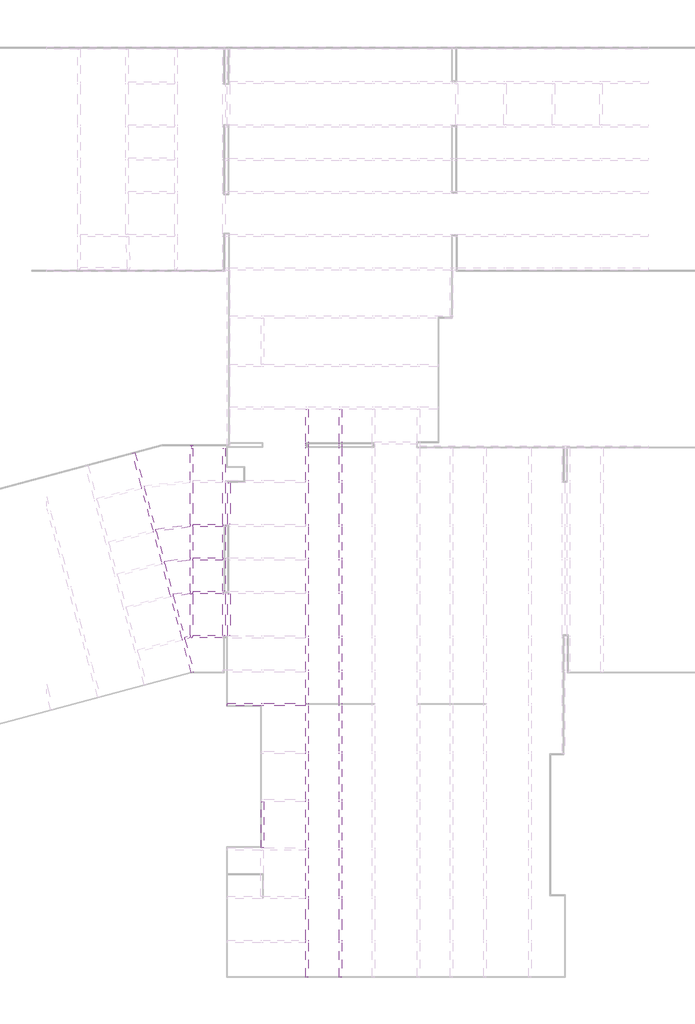
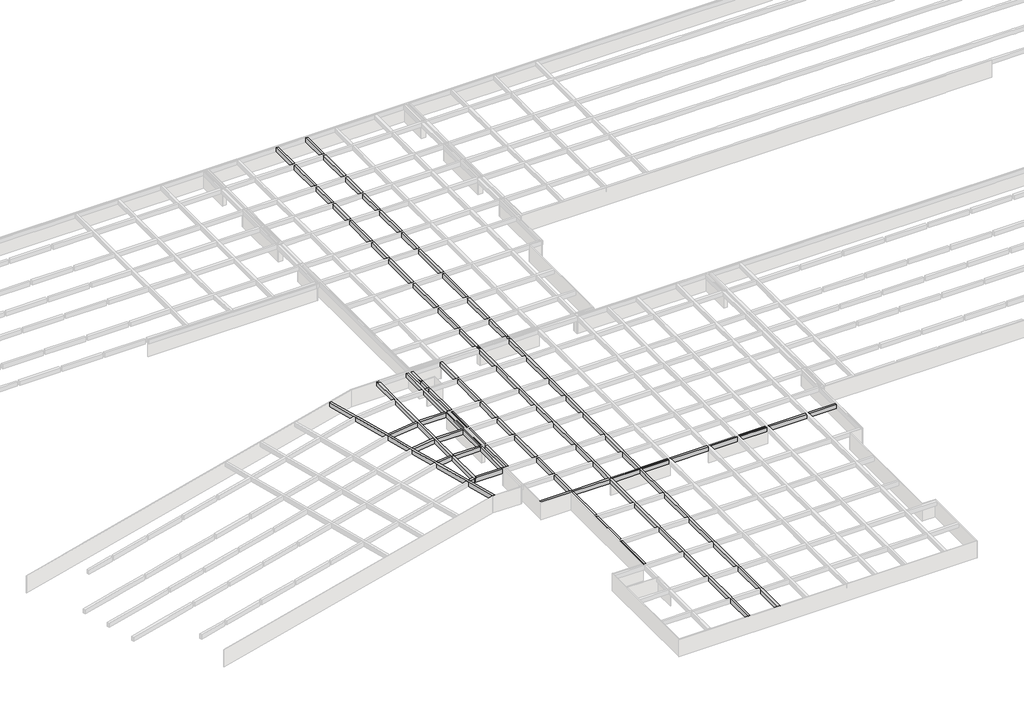
# One storey, part 7 of 14: 19 beams.
"""IFC4 building model written with IfcOpenShell, lengths in millimetres."""

import ifcopenshell
import ifcopenshell.guid

model = None  # the IFC model being written
_history = None  # IfcOwnerHistory: only IFC2X3 demands one
_inside = {}  # id of a spatial element -> (the spatial element, [elements in it])
_under = {}  # id of a project, library or spatial element -> (it, [spatial elements below it])
_declared = {}  # id of a project -> (the project, [libraries it declares])
_typed = {}  # id of a type object -> (the type object, [elements of that type])
_made_of = {}  # id of a material, layer set ... -> (it, [elements and type objects made of it])


def new_model(schema):
    """Start an empty IFC model of exactly this schema.

    Asked for "IFC4X3", IfcOpenShell would pick the latest addendum, in which some entities
    have other attributes; the version numbers below select the first issue.
    IFC2X3 requires an IfcOwnerHistory on every rooted entity: one is made here for all.
    """
    global model, _history
    if schema == "IFC4X3":
        model = ifcopenshell.file(schema_version=(4, 3, 0, 0))
    else:
        model = ifcopenshell.file(schema=schema)
    _inside.clear()
    _under.clear()
    _declared.clear()
    _typed.clear()
    _made_of.clear()
    _history = None
    if model.schema == "IFC2X3":
        org = make("IfcOrganization", Name="unknown")
        user = make(
            "IfcPersonAndOrganization",
            ThePerson=make("IfcPerson", FamilyName="unknown"),
            TheOrganization=org,
        )
        app = make(
            "IfcApplication",
            ApplicationDeveloper=org,
            Version="unknown",
            ApplicationFullName="unknown",
            ApplicationIdentifier="unknown",
        )
        _history = make(
            "IfcOwnerHistory",
            OwningUser=user,
            OwningApplication=app,
            ChangeAction="ADDED",
            CreationDate=0,
        )
    return model


def make(cls, **values):
    """One entity of the class cls with the attributes given. An attribute that is None is left unset."""
    return model.create_entity(
        cls, **{name: value for name, value in values.items() if value is not None}
    )


def rooted(cls, **values):
    """An entity with a GlobalId (a new one), such as an element, a storey or a relation."""
    return make(cls, GlobalId=ifcopenshell.guid.new(), OwnerHistory=_history, **values)


def si_unit(unit_type, name, prefix=None):
    """IfcSIUnit, for example si_unit("LENGTHUNIT", "METRE", prefix="MILLI")."""
    return make("IfcSIUnit", UnitType=unit_type, Prefix=prefix, Name=name)


def assignment(units):
    """IfcUnitAssignment: the units of a project."""
    return None if units is None else make("IfcUnitAssignment", Units=units)


def point(xyz):
    """IfcCartesianPoint."""
    return None if xyz is None else make("IfcCartesianPoint", Coordinates=xyz)


def direction(xyz):
    """IfcDirection."""
    return None if xyz is None else make("IfcDirection", DirectionRatios=xyz)


def frame(location, z_axis=None, x_axis=None):
    """IfcAxis2Placement3D, a coordinate frame: its origin and axes. An axis left out is left unset."""
    return make(
        "IfcAxis2Placement3D",
        Location=point(location),
        Axis=direction(z_axis),
        RefDirection=direction(x_axis),
    )


def origin():
    """The frame at (0, 0, 0) with its axes left unset."""
    return frame((0.0, 0.0, 0.0))


def place(relative_to, where):
    """IfcLocalPlacement: puts the frame where relative to a parent placement (None: the world)."""
    return make(
        "IfcLocalPlacement", PlacementRelTo=relative_to, RelativePlacement=where
    )


def context(
    kind, dimensions, precision=None, world=None, true_north=None, identifier=None
):
    """IfcGeometricRepresentationContext, for example the 3D "Model" context."""
    return make(
        "IfcGeometricRepresentationContext",
        ContextIdentifier=identifier,
        ContextType=kind,
        CoordinateSpaceDimension=dimensions,
        Precision=precision,
        WorldCoordinateSystem=world,
        TrueNorth=true_north,
    )


def project(units=None, contexts=None):
    """IfcProject with its units and contexts."""
    return rooted(
        "IfcProject",
        Name="project",
        RepresentationContexts=contexts,
        UnitsInContext=assignment(units),
    )


def spatial(cls, under=None, at=None, **own):
    """A site, building, storey or space (cls), placed at a placement, below another one or the project."""
    s = rooted(cls, ObjectPlacement=at, **own)
    if under is not None:
        _under.setdefault(under.id(), (under, []))[1].append(s)
    return s


def polyline(points):
    """IfcPolyline through the points."""
    return make("IfcPolyline", Points=[point(p) for p in points])


def outline(outer, holes=None, kind="AREA"):
    """IfcArbitraryClosedProfileDef: a profile drawn as a closed curve; with holes, ...WithVoids."""
    if holes is None:
        return make("IfcArbitraryClosedProfileDef", ProfileType=kind, OuterCurve=outer)
    return make(
        "IfcArbitraryProfileDefWithVoids",
        ProfileType=kind,
        OuterCurve=outer,
        InnerCurves=holes,
    )


def extrude(swept, where, along, depth):
    """IfcExtrudedAreaSolid: the profile swept, set in the frame where, extruded along a direction by depth."""
    return make(
        "IfcExtrudedAreaSolid",
        SweptArea=swept,
        Position=where,
        ExtrudedDirection=direction(along),
        Depth=depth,
    )


def faces_of(points, faces, orient=None, outer=None):
    """IfcFace entities. A face is a list of loops; a loop is a list of indices into points, from 0.

    orient and outer hold one flag for each loop. By default every Orientation is true, the
    first loop of a face is its IfcFaceOuterBound and the others are IfcFaceBound.
    """
    made = []
    for i, loops in enumerate(faces):
        bounds = []
        for j, loop in enumerate(loops):
            is_outer = j == 0 if outer is None else outer[i][j]
            bounds.append(
                make(
                    "IfcFaceOuterBound" if is_outer else "IfcFaceBound",
                    Bound=make("IfcPolyLoop", Polygon=[points[k] for k in loop]),
                    Orientation=True if orient is None else orient[i][j],
                )
            )
        made.append(make("IfcFace", Bounds=bounds))
    return made


def faceted_brep(points, faces, orient=None, outer=None, voids=None):
    """IfcFacetedBrep: a solid bounded by flat faces; with voids (closed shells), ...WithVoids."""
    shared = [point(p) for p in points]
    hull = make("IfcClosedShell", CfsFaces=faces_of(shared, faces, orient, outer))
    if voids is None:
        return make("IfcFacetedBrep", Outer=hull)
    return make(
        "IfcFacetedBrepWithVoids",
        Outer=hull,
        Voids=[
            make(cls, CfsFaces=faces_of(shared, fs, o, b)) for cls, fs, o, b in voids
        ],
    )


def shape(context_of_items, identifier, shape_type, items):
    """IfcShapeRepresentation: the items that make up one representation, for example the "Body"."""
    return make(
        "IfcShapeRepresentation",
        ContextOfItems=context_of_items,
        RepresentationIdentifier=identifier,
        RepresentationType=shape_type,
        Items=items,
    )


def made_of(thing, what):
    """Note that an element or type object is made of a material, layer set ...; save() writes the relation."""
    if what is not None:
        _made_of.setdefault(what.id(), (what, []))[1].append(thing)
    return thing


def element(
    cls,
    number,
    at=None,
    inside=None,
    cuts=None,
    type_object=None,
    material=None,
    context=None,
    identifier="Body",
    shape_type=None,
    held_by="IfcProductDefinitionShape",
    body=None,
    shapes=None,
    **own,
):
    """One element of the class cls, such as IfcWall. Its Tag is "e" and its number.

    at: its placement. inside: the storey or other place that contains it. cuts: it is an
    opening in that element (IfcRelVoidsElement). A single representation is given by context,
    identifier, shape_type and body (its items); several are given by shapes. held_by: the class
    of the entity that holds the representations. save() writes the other relations.
    """
    e = rooted(cls, Tag="e%d" % number, ObjectPlacement=at, **own)
    if body is not None:
        shapes = [shape(context, identifier, shape_type, body)]
    if shapes is not None:
        e.Representation = make(held_by, Representations=shapes)
    if inside is not None:
        _inside.setdefault(inside.id(), (inside, []))[1].append(e)
    if cuts is not None:
        rooted(
            "IfcRelVoidsElement", RelatingBuildingElement=cuts, RelatedOpeningElement=e
        )
    if type_object is not None:
        _typed.setdefault(type_object.id(), (type_object, []))[1].append(e)
    return made_of(e, material)


def aggregate(whole, parts):
    """IfcRelAggregates: a whole, such as a stair, and the parts it consists of."""
    return rooted("IfcRelAggregates", RelatingObject=whole, RelatedObjects=parts)


def save(model, path):
    """Write the relations noted so far, then the file.

    IfcRelAggregates (storeys below a building ...), IfcRelContainedInSpatialStructure (elements
    in a storey), IfcRelDefinesByType, IfcRelAssociatesMaterial and IfcRelDeclares: one each for
    every whole, place, type object, material and project.
    """
    for whole, parts in _under.values():
        aggregate(whole, parts)
    for where, things in _inside.values():
        rooted(
            "IfcRelContainedInSpatialStructure",
            RelatedElements=things,
            RelatingStructure=where,
        )
    for kind, things in _typed.values():
        rooted("IfcRelDefinesByType", RelatedObjects=things, RelatingType=kind)
    for what, things in _made_of.values():
        rooted("IfcRelAssociatesMaterial", RelatedObjects=things, RelatingMaterial=what)
    for by, libraries in _declared.values():
        rooted("IfcRelDeclares", RelatingContext=by, RelatedDefinitions=libraries)
    model.write(path)


model = new_model("IFC4")

# Units and contexts
model_context = context("Model", 3, world=origin())
ifc_project = project(units=[si_unit("LENGTHUNIT", "METRE", prefix="MILLI")], contexts=[model_context])

# Site, building, storey
site = spatial("IfcSite", under=ifc_project)
building = spatial("IfcBuilding", under=site)
storey = spatial("IfcBuildingStorey", under=building, Name="户型图", Elevation=0.0)

# Beams
placement = place(None, origin())
element("IfcBeam", 1, ObjectType="混凝土 - 矩形梁 : KL_beam", at=placement, inside=storey, context=model_context, shape_type="Brep", body=[
    faceted_brep([(26321.5607309, -267473.0312098, 3300.0), (25921.5607309, -267473.0312098, 3300.0), (25921.5607309, -267473.0312098, 2500.0), (26321.5607309, -267473.0312098, 2500.0), (26321.5607309, -261891.8929199, 3300.0), (26321.5607309, -261491.8929199, 3300.0), (26321.5607309, -254823.1116625, 3300.0), (26321.5607309, -254423.1116625, 3300.0), (26321.5607309, -247008.950757, 3300.0), (26321.5607309, -246608.950757, 3300.0), (26321.5607309, -239178.950757, 3300.0), (26321.5607309, -238778.950757, 3300.0), (26321.5607309, -231409.1116625, 3300.0), (26321.5607309, -231009.1116625, 3300.0), (26321.5607309, -223621.814057, 3300.0), (26321.5607309, -223221.814057, 3300.0), (26321.5607309, -218208.950757, 3300.0), (26321.5607309, -217808.950757, 3300.0), (26321.5607309, -212708.950757, 3300.0), (26321.5607309, -212308.950757, 3300.0), (26321.5607309, -205576.1028577, 3300.0), (26321.5607309, -205176.1028577, 3300.0), (26321.5607309, -200154.952508, 3300.0), (26321.5607309, -199754.952508, 3300.0), (26321.5607309, -194741.3993539, 3300.0), (26321.5607309, -194341.3993539, 3300.0), (26321.5607309, -187598.950757, 3300.0), (26321.5607309, -187198.950757, 3300.0), (26321.5607309, -182068.950757, 3300.0), (26321.5607309, -181668.950757, 3300.0), (26321.5607309, -181394.9655707, 3300.0), (26321.5607309, -180994.9655707, 3300.0), (26321.5607309, -175717.1358924, 3300.0), (25921.5607309, -175717.1358924, 3300.0), (25921.5607309, -180994.9655707, 3300.0), (25921.5607309, -181394.9655707, 3300.0), (25921.5607309, -181668.950757, 3300.0), (25921.5607309, -182068.950757, 3300.0), (25921.5607309, -187198.950757, 3300.0), (25921.5607309, -187598.950757, 3300.0), (25921.5607309, -194341.3993539, 3300.0), (25921.5607309, -194741.3993539, 3300.0), (25921.5607309, -199754.952508, 3300.0), (25921.5607309, -200154.952508, 3300.0), (25921.5607309, -205176.1028577, 3300.0), (25921.5607309, -205576.1028577, 3300.0), (25921.5607309, -212308.950757, 3300.0), (25921.5607309, -212708.950757, 3300.0), (25921.5607309, -217808.950757, 3300.0), (25921.5607309, -218208.950757, 3300.0), (25921.5607309, -223221.814057, 3300.0), (25921.5607309, -223621.814057, 3300.0), (25921.5607309, -231009.1116625, 3300.0), (25921.5607309, -231409.1116625, 3300.0), (25921.5607309, -238778.950757, 3300.0), (25921.5607309, -239178.950757, 3300.0), (25921.5607309, -246608.950757, 3300.0), (25921.5607309, -247008.950757, 3300.0), (25921.5607309, -254423.1116625, 3300.0), (25921.5607309, -254823.1116625, 3300.0), (25921.5607309, -261491.8929199, 3300.0), (25921.5607309, -261891.8929199, 3300.0), (25921.5607309, -175717.1358924, 2500.0), (25921.5607309, -180994.9655707, 2500.0), (25921.5607309, -181394.9655707, 2500.0), (25921.5607309, -181668.950757, 2500.0), (25921.5607309, -182068.950757, 2500.0), (25921.5607309, -187198.950757, 2500.0), (25921.5607309, -187598.950757, 2500.0), (25921.5607309, -194341.3993539, 2500.0), (25921.5607309, -194741.3993539, 2500.0), (25921.5607309, -199754.952508, 2500.0), (25921.5607309, -200154.952508, 2500.0), (25921.5607309, -205176.1028577, 2500.0), (25921.5607309, -205576.1028577, 2500.0), (25921.5607309, -212308.950757, 2500.0), (25921.5607309, -212708.950757, 2500.0), (25921.5607309, -217808.950757, 2500.0), (25921.5607309, -218208.950757, 2500.0), (25921.5607309, -223221.814057, 2500.0), (25921.5607309, -223621.814057, 2500.0), (25921.5607309, -231009.1116625, 2500.0), (25921.5607309, -231409.1116625, 2500.0), (25921.5607309, -238778.950757, 2500.0), (25921.5607309, -239178.950757, 2500.0), (25921.5607309, -246608.950757, 2500.0), (25921.5607309, -247008.950757, 2500.0), (25921.5607309, -254423.1116625, 2500.0), (25921.5607309, -254823.1116625, 2500.0), (25921.5607309, -261491.8929199, 2500.0), (25921.5607309, -261891.8929199, 2500.0), (26321.5607309, -175717.1358924, 2500.0), (26321.5607309, -180994.9655707, 2500.0), (26321.5607309, -181394.9655707, 2500.0), (26321.5607309, -181668.950757, 2500.0), (26321.5607309, -182068.950757, 2500.0), (26321.5607309, -187198.950757, 2500.0), (26321.5607309, -187598.950757, 2500.0), (26321.5607309, -194341.3993539, 2500.0), (26321.5607309, -194741.3993539, 2500.0), (26321.5607309, -199754.952508, 2500.0), (26321.5607309, -200154.952508, 2500.0), (26321.5607309, -205176.1028577, 2500.0), (26321.5607309, -205576.1028577, 2500.0), (26321.5607309, -212308.950757, 2500.0), (26321.5607309, -212708.950757, 2500.0), (26321.5607309, -217808.950757, 2500.0), (26321.5607309, -218208.950757, 2500.0), (26321.5607309, -223221.814057, 2500.0), (26321.5607309, -223621.814057, 2500.0), (26321.5607309, -231009.1116625, 2500.0), (26321.5607309, -231409.1116625, 2500.0), (26321.5607309, -238778.950757, 2500.0), (26321.5607309, -239178.950757, 2500.0), (26321.5607309, -246608.950757, 2500.0), (26321.5607309, -247008.950757, 2500.0), (26321.5607309, -254423.1116625, 2500.0), (26321.5607309, -254823.1116625, 2500.0), (26321.5607309, -261491.8929199, 2500.0), (26321.5607309, -261891.8929199, 2500.0)], [[[0, 1, 2, 3]], [[1, 0, 4, 5, 6, 7, 8, 9, 10, 11, 12, 13, 14, 15, 16, 17, 18, 19, 20, 21, 22, 23, 24, 25, 26, 27, 28, 29, 30, 31, 32, 33, 34, 35, 36, 37, 38, 39, 40, 41, 42, 43, 44, 45, 46, 47, 48, 49, 50, 51, 52, 53, 54, 55, 56, 57, 58, 59, 60, 61]], [[2, 1, 61, 60, 59, 58, 57, 56, 55, 54, 53, 52, 51, 50, 49, 48, 47, 46, 45, 44, 43, 42, 41, 40, 39, 38, 37, 36, 35, 34, 33, 62, 63, 64, 65, 66, 67, 68, 69, 70, 71, 72, 73, 74, 75, 76, 77, 78, 79, 80, 81, 82, 83, 84, 85, 86, 87, 88, 89, 90]], [[3, 2, 90, 89, 88, 87, 86, 85, 84, 83, 82, 81, 80, 79, 78, 77, 76, 75, 74, 73, 72, 71, 70, 69, 68, 67, 66, 65, 64, 63, 62, 91, 92, 93, 94, 95, 96, 97, 98, 99, 100, 101, 102, 103, 104, 105, 106, 107, 108, 109, 110, 111, 112, 113, 114, 115, 116, 117, 118, 119]], [[0, 3, 119, 118, 117, 116, 115, 114, 113, 112, 111, 110, 109, 108, 107, 106, 105, 104, 103, 102, 101, 100, 99, 98, 97, 96, 95, 94, 93, 92, 91, 32, 31, 30, 29, 28, 27, 26, 25, 24, 23, 22, 21, 20, 19, 18, 17, 16, 15, 14, 13, 12, 11, 10, 9, 8, 7, 6, 5, 4]], [[33, 32, 91, 62]]]),
    faceted_brep([(25921.5607309, -123197.8127788, 3300.0), (26321.5607309, -123197.8127788, 3300.0), (26321.5607309, -123197.8127788, 2500.0), (25921.5607309, -123197.8127788, 2500.0), (26321.5607309, -129780.0179086, 3300.0), (25921.5607309, -129780.0179086, 3300.0), (25921.5607309, -129780.0179086, 2500.0), (26321.5607309, -129780.0179086, 2500.0)], [[[0, 1, 2, 3]], [[4, 5, 6, 7]], [[1, 0, 5, 4]], [[0, 3, 6, 5]], [[3, 2, 7, 6]], [[2, 1, 4, 7]]]),
    faceted_brep([(26321.5607309, -122797.8127788, 3300.0), (25921.5607309, -122797.8127788, 3300.0), (25921.5607309, -122797.8127788, 2500.0), (26321.5607309, -122797.8127788, 2500.0), (26321.5607309, -117558.950757, 3300.0), (25921.5607309, -117558.950757, 3300.0), (25921.5607309, -117558.950757, 2500.0), (26321.5607309, -117558.950757, 2500.0)], [[[0, 1, 2, 3]], [[1, 0, 4, 5]], [[2, 1, 5, 6]], [[3, 2, 6, 7]], [[0, 3, 7, 4]], [[5, 4, 7, 6]]]),
    faceted_brep([(25921.5607309, -130180.0179086, 3300.0), (26321.5607309, -130180.0179086, 3300.0), (26321.5607309, -130180.0179086, 2500.0), (25921.5607309, -130180.0179086, 2500.0), (26321.5607309, -135180.0179086, 3300.0), (25921.5607309, -135180.0179086, 3300.0), (25921.5607309, -135180.0179086, 2500.0), (26321.5607309, -135180.0179086, 2500.0)], [[[0, 1, 2, 3]], [[4, 5, 6, 7]], [[1, 0, 5, 4]], [[0, 3, 6, 5]], [[3, 2, 7, 6]], [[2, 1, 4, 7]]]),
    faceted_brep([(25921.5607309, -135580.0179086, 3300.0), (26321.5607309, -135580.0179086, 3300.0), (26321.5607309, -135580.0179086, 2500.0), (25921.5607309, -135580.0179086, 2500.0), (26321.5607309, -140520.0179086, 3300.0), (25921.5607309, -140520.0179086, 3300.0), (25921.5607309, -140520.0179086, 2500.0), (26321.5607309, -140520.0179086, 2500.0)], [[[0, 1, 2, 3]], [[4, 5, 6, 7]], [[1, 0, 5, 4]], [[0, 3, 6, 5]], [[3, 2, 7, 6]], [[2, 1, 4, 7]]]),
    faceted_brep([(25921.5607309, -140920.0179086, 3300.0), (26321.5607309, -140920.0179086, 3300.0), (26321.5607309, -140920.0179086, 2500.0), (25921.5607309, -140920.0179086, 2500.0), (26321.5607309, -147499.284307, 3300.0), (25921.5607309, -147499.284307, 3300.0), (25921.5607309, -147499.284307, 2500.0), (26321.5607309, -147499.284307, 2500.0)], [[[0, 1, 2, 3]], [[4, 5, 6, 7]], [[1, 0, 5, 4]], [[0, 3, 6, 5]], [[3, 2, 7, 6]], [[2, 1, 4, 7]]]),
    faceted_brep([(25921.5607309, -147899.284307, 3300.0), (26321.5607309, -147899.284307, 3300.0), (26321.5607309, -147899.284307, 2500.0), (25921.5607309, -147899.284307, 2500.0), (26321.5607309, -152899.284307, 3300.0), (25921.5607309, -152899.284307, 3300.0), (25921.5607309, -152899.284307, 2500.0), (26321.5607309, -152899.284307, 2500.0)], [[[0, 1, 2, 3]], [[4, 5, 6, 7]], [[1, 0, 5, 4]], [[0, 3, 6, 5]], [[3, 2, 7, 6]], [[2, 1, 4, 7]]]),
    faceted_brep([(25921.5607309, -153299.284307, 3300.0), (26321.5607309, -153299.284307, 3300.0), (26321.5607309, -153299.284307, 2500.0), (25921.5607309, -153299.284307, 2500.0), (26321.5607309, -160620.767119, 3300.0), (25921.5607309, -160620.767119, 3300.0), (25921.5607309, -160620.767119, 2500.0), (26321.5607309, -160620.767119, 2500.0)], [[[0, 1, 2, 3]], [[4, 5, 6, 7]], [[1, 0, 5, 4]], [[0, 3, 6, 5]], [[3, 2, 7, 6]], [[2, 1, 4, 7]]]),
    faceted_brep([(25921.5607309, -161020.767119, 3300.0), (26321.5607309, -161020.767119, 3300.0), (26321.5607309, -161020.767119, 2500.0), (25921.5607309, -161020.767119, 2500.0), (26321.5607309, -168501.0793872, 3300.0), (25921.5607309, -168501.0793872, 3300.0), (25921.5607309, -168501.0793872, 2500.0), (26321.5607309, -168501.0793872, 2500.0)], [[[0, 1, 2, 3]], [[4, 5, 6, 7]], [[1, 0, 5, 4]], [[0, 3, 6, 5]], [[3, 2, 7, 6]], [[2, 1, 4, 7]]]),
    faceted_brep([(25921.5607309, -168901.0793872, 3300.0), (26321.5607309, -168901.0793872, 3300.0), (26321.5607309, -168901.0793872, 2500.0), (25921.5607309, -168901.0793872, 2500.0), (26321.5607309, -175317.1358924, 3300.0), (25921.5607309, -175317.1358924, 3300.0), (25921.5607309, -175317.1358924, 2500.0), (26321.5607309, -175317.1358924, 2500.0)], [[[0, 1, 2, 3]], [[4, 5, 6, 7]], [[1, 0, 5, 4]], [[0, 3, 6, 5]], [[3, 2, 7, 6]], [[2, 1, 4, 7]]]),
])
element("IfcBeam", 2, ObjectType="混凝土 - 矩形梁 : KL_beam", at=placement, inside=storey, context=model_context, shape_type="Brep", body=[
    faceted_brep([(31351.9066405, -267473.0312098, 3300.0), (31351.9066405, -267473.0312098, 2500.0), (31751.9066405, -267473.0312098, 2500.0), (31751.9066405, -267473.0312098, 3300.0), (31351.9066405, -175717.1358924, 3300.0), (31751.9066405, -175717.1358924, 3300.0), (31751.9066405, -175717.1358924, 2500.0), (31351.9066405, -175717.1358924, 2500.0), (31751.9066405, -261891.8929199, 3300.0), (31751.9066405, -261491.8929199, 3300.0), (31751.9066405, -254823.1116625, 3300.0), (31751.9066405, -254423.1116625, 3300.0), (31751.9066405, -247008.950757, 3300.0), (31751.9066405, -246608.950757, 3300.0), (31751.9066405, -239178.950757, 3300.0), (31751.9066405, -238778.950757, 3300.0), (31751.9066405, -231409.1116625, 3300.0), (31751.9066405, -231009.1116625, 3300.0), (31751.9066405, -223621.814057, 3300.0), (31751.9066405, -223221.814057, 3300.0), (31751.9066405, -218208.950757, 3300.0), (31751.9066405, -217808.950757, 3300.0), (31751.9066405, -212708.950757, 3300.0), (31751.9066405, -212308.950757, 3300.0), (31751.9066405, -205576.1028577, 3300.0), (31751.9066405, -205176.1028577, 3300.0), (31751.9066405, -200154.952508, 3300.0), (31751.9066405, -199754.952508, 3300.0), (31751.9066405, -194741.3993539, 3300.0), (31751.9066405, -194341.3993539, 3300.0), (31751.9066405, -187598.950757, 3300.0), (31751.9066405, -187198.950757, 3300.0), (31751.9066405, -182068.950757, 3300.0), (31751.9066405, -181668.950757, 3300.0), (31751.9066405, -181394.9655707, 3300.0), (31751.9066405, -180994.9655707, 3300.0), (31351.9066405, -180994.9655707, 3300.0), (31351.9066405, -181394.9655707, 3300.0), (31351.9066405, -181668.950757, 3300.0), (31351.9066405, -182068.950757, 3300.0), (31351.9066405, -187198.950757, 3300.0), (31351.9066405, -187598.950757, 3300.0), (31351.9066405, -194341.3993539, 3300.0), (31351.9066405, -194741.3993539, 3300.0), (31351.9066405, -199754.952508, 3300.0), (31351.9066405, -200154.952508, 3300.0), (31351.9066405, -205176.1028577, 3300.0), (31351.9066405, -205576.1028577, 3300.0), (31351.9066405, -212308.950757, 3300.0), (31351.9066405, -212708.950757, 3300.0), (31351.9066405, -217808.950757, 3300.0), (31351.9066405, -218208.950757, 3300.0), (31351.9066405, -223221.814057, 3300.0), (31351.9066405, -223621.814057, 3300.0), (31351.9066405, -231009.1116625, 3300.0), (31351.9066405, -231409.1116625, 3300.0), (31351.9066405, -238778.950757, 3300.0), (31351.9066405, -239178.950757, 3300.0), (31351.9066405, -246608.950757, 3300.0), (31351.9066405, -247008.950757, 3300.0), (31351.9066405, -254423.1116625, 3300.0), (31351.9066405, -254823.1116625, 3300.0), (31351.9066405, -261491.8929199, 3300.0), (31351.9066405, -261891.8929199, 3300.0), (31751.9066405, -261891.8929199, 2500.0), (31751.9066405, -261491.8929199, 2500.0), (31751.9066405, -254823.1116625, 2500.0), (31751.9066405, -254423.1116625, 2500.0), (31751.9066405, -247008.950757, 2500.0), (31751.9066405, -246608.950757, 2500.0), (31751.9066405, -239178.950757, 2500.0), (31751.9066405, -238778.950757, 2500.0), (31751.9066405, -231409.1116625, 2500.0), (31751.9066405, -231009.1116625, 2500.0), (31751.9066405, -223621.814057, 2500.0), (31751.9066405, -223221.814057, 2500.0), (31751.9066405, -218208.950757, 2500.0), (31751.9066405, -217808.950757, 2500.0), (31751.9066405, -212708.950757, 2500.0), (31751.9066405, -212308.950757, 2500.0), (31751.9066405, -205576.1028577, 2500.0), (31751.9066405, -205176.1028577, 2500.0), (31751.9066405, -200154.952508, 2500.0), (31751.9066405, -199754.952508, 2500.0), (31751.9066405, -194741.3993539, 2500.0), (31751.9066405, -194341.3993539, 2500.0), (31751.9066405, -187598.950757, 2500.0), (31751.9066405, -187198.950757, 2500.0), (31751.9066405, -182068.950757, 2500.0), (31751.9066405, -181668.950757, 2500.0), (31751.9066405, -181394.9655707, 2500.0), (31751.9066405, -180994.9655707, 2500.0), (31351.9066405, -261891.8929199, 2500.0), (31351.9066405, -261491.8929199, 2500.0), (31351.9066405, -254823.1116625, 2500.0), (31351.9066405, -254423.1116625, 2500.0), (31351.9066405, -247008.950757, 2500.0), (31351.9066405, -246608.950757, 2500.0), (31351.9066405, -239178.950757, 2500.0), (31351.9066405, -238778.950757, 2500.0), (31351.9066405, -231409.1116625, 2500.0), (31351.9066405, -231009.1116625, 2500.0), (31351.9066405, -223621.814057, 2500.0), (31351.9066405, -223221.814057, 2500.0), (31351.9066405, -218208.950757, 2500.0), (31351.9066405, -217808.950757, 2500.0), (31351.9066405, -212708.950757, 2500.0), (31351.9066405, -212308.950757, 2500.0), (31351.9066405, -205576.1028577, 2500.0), (31351.9066405, -205176.1028577, 2500.0), (31351.9066405, -200154.952508, 2500.0), (31351.9066405, -199754.952508, 2500.0), (31351.9066405, -194741.3993539, 2500.0), (31351.9066405, -194341.3993539, 2500.0), (31351.9066405, -187598.950757, 2500.0), (31351.9066405, -187198.950757, 2500.0), (31351.9066405, -182068.950757, 2500.0), (31351.9066405, -181668.950757, 2500.0), (31351.9066405, -181394.9655707, 2500.0), (31351.9066405, -180994.9655707, 2500.0)], [[[0, 1, 2, 3]], [[4, 5, 6, 7]], [[0, 3, 8, 9, 10, 11, 12, 13, 14, 15, 16, 17, 18, 19, 20, 21, 22, 23, 24, 25, 26, 27, 28, 29, 30, 31, 32, 33, 34, 35, 5, 4, 36, 37, 38, 39, 40, 41, 42, 43, 44, 45, 46, 47, 48, 49, 50, 51, 52, 53, 54, 55, 56, 57, 58, 59, 60, 61, 62, 63]], [[3, 2, 64, 65, 66, 67, 68, 69, 70, 71, 72, 73, 74, 75, 76, 77, 78, 79, 80, 81, 82, 83, 84, 85, 86, 87, 88, 89, 90, 91, 6, 5, 35, 34, 33, 32, 31, 30, 29, 28, 27, 26, 25, 24, 23, 22, 21, 20, 19, 18, 17, 16, 15, 14, 13, 12, 11, 10, 9, 8]], [[2, 1, 92, 93, 94, 95, 96, 97, 98, 99, 100, 101, 102, 103, 104, 105, 106, 107, 108, 109, 110, 111, 112, 113, 114, 115, 116, 117, 118, 119, 7, 6, 91, 90, 89, 88, 87, 86, 85, 84, 83, 82, 81, 80, 79, 78, 77, 76, 75, 74, 73, 72, 71, 70, 69, 68, 67, 66, 65, 64]], [[1, 0, 63, 62, 61, 60, 59, 58, 57, 56, 55, 54, 53, 52, 51, 50, 49, 48, 47, 46, 45, 44, 43, 42, 41, 40, 39, 38, 37, 36, 4, 7, 119, 118, 117, 116, 115, 114, 113, 112, 111, 110, 109, 108, 107, 106, 105, 104, 103, 102, 101, 100, 99, 98, 97, 96, 95, 94, 93, 92]]]),
    faceted_brep([(31351.9066405, -122797.8127788, 3300.0), (31751.9066405, -122797.8127788, 3300.0), (31751.9066405, -117558.950757, 3300.0), (31351.9066405, -117558.950757, 3300.0), (31751.9066405, -122797.8127788, 2500.0), (31751.9066405, -117558.950757, 2500.0), (31351.9066405, -122797.8127788, 2500.0), (31351.9066405, -117558.950757, 2500.0)], [[[0, 1, 2, 3]], [[1, 4, 5, 2]], [[4, 6, 7, 5]], [[6, 0, 3, 7]], [[1, 0, 6, 4]], [[3, 2, 5, 7]]]),
    faceted_brep([(31351.9066405, -123197.8127788, 3300.0), (31751.9066405, -123197.8127788, 3300.0), (31751.9066405, -123197.8127788, 2500.0), (31351.9066405, -123197.8127788, 2500.0), (31351.9066405, -129780.0179086, 3300.0), (31751.9066405, -129780.0179086, 3300.0), (31751.9066405, -129780.0179086, 2500.0), (31351.9066405, -129780.0179086, 2500.0)], [[[0, 1, 2, 3]], [[1, 0, 4, 5]], [[2, 1, 5, 6]], [[3, 2, 6, 7]], [[0, 3, 7, 4]], [[5, 4, 7, 6]]]),
    faceted_brep([(31351.9066405, -130180.0179086, 3300.0), (31751.9066405, -130180.0179086, 3300.0), (31751.9066405, -130180.0179086, 2500.0), (31351.9066405, -130180.0179086, 2500.0), (31351.9066405, -135180.0179086, 3300.0), (31751.9066405, -135180.0179086, 3300.0), (31751.9066405, -135180.0179086, 2500.0), (31351.9066405, -135180.0179086, 2500.0)], [[[0, 1, 2, 3]], [[1, 0, 4, 5]], [[2, 1, 5, 6]], [[3, 2, 6, 7]], [[0, 3, 7, 4]], [[5, 4, 7, 6]]]),
    faceted_brep([(31351.9066405, -135580.0179086, 3300.0), (31751.9066405, -135580.0179086, 3300.0), (31751.9066405, -135580.0179086, 2500.0), (31351.9066405, -135580.0179086, 2500.0), (31351.9066405, -140520.0179086, 3300.0), (31751.9066405, -140520.0179086, 3300.0), (31751.9066405, -140520.0179086, 2500.0), (31351.9066405, -140520.0179086, 2500.0)], [[[0, 1, 2, 3]], [[1, 0, 4, 5]], [[2, 1, 5, 6]], [[3, 2, 6, 7]], [[0, 3, 7, 4]], [[5, 4, 7, 6]]]),
    faceted_brep([(31351.9066405, -140920.0179086, 3300.0), (31751.9066405, -140920.0179086, 3300.0), (31751.9066405, -140920.0179086, 2500.0), (31351.9066405, -140920.0179086, 2500.0), (31351.9066405, -147499.284307, 3300.0), (31751.9066405, -147499.284307, 3300.0), (31751.9066405, -147499.284307, 2500.0), (31351.9066405, -147499.284307, 2500.0)], [[[0, 1, 2, 3]], [[1, 0, 4, 5]], [[2, 1, 5, 6]], [[3, 2, 6, 7]], [[0, 3, 7, 4]], [[5, 4, 7, 6]]]),
    faceted_brep([(31351.9066405, -147899.284307, 3300.0), (31751.9066405, -147899.284307, 3300.0), (31751.9066405, -147899.284307, 2500.0), (31351.9066405, -147899.284307, 2500.0), (31351.9066405, -152899.284307, 3300.0), (31751.9066405, -152899.284307, 3300.0), (31751.9066405, -152899.284307, 2500.0), (31351.9066405, -152899.284307, 2500.0)], [[[0, 1, 2, 3]], [[1, 0, 4, 5]], [[2, 1, 5, 6]], [[3, 2, 6, 7]], [[0, 3, 7, 4]], [[5, 4, 7, 6]]]),
    faceted_brep([(31351.9066405, -153299.284307, 3300.0), (31751.9066405, -153299.284307, 3300.0), (31751.9066405, -153299.284307, 2500.0), (31351.9066405, -153299.284307, 2500.0), (31351.9066405, -160620.767119, 3300.0), (31751.9066405, -160620.767119, 3300.0), (31751.9066405, -160620.767119, 2500.0), (31351.9066405, -160620.767119, 2500.0)], [[[0, 1, 2, 3]], [[1, 0, 4, 5]], [[2, 1, 5, 6]], [[3, 2, 6, 7]], [[0, 3, 7, 4]], [[5, 4, 7, 6]]]),
    faceted_brep([(31351.9066405, -161020.767119, 3300.0), (31751.9066405, -161020.767119, 3300.0), (31751.9066405, -161020.767119, 2500.0), (31351.9066405, -161020.767119, 2500.0), (31351.9066405, -168501.0793872, 3300.0), (31751.9066405, -168501.0793872, 3300.0), (31751.9066405, -168501.0793872, 2500.0), (31351.9066405, -168501.0793872, 2500.0)], [[[0, 1, 2, 3]], [[1, 0, 4, 5]], [[2, 1, 5, 6]], [[3, 2, 6, 7]], [[0, 3, 7, 4]], [[5, 4, 7, 6]]]),
    faceted_brep([(31351.9066405, -168901.0793872, 3300.0), (31751.9066405, -168901.0793872, 3300.0), (31751.9066405, -168901.0793872, 2500.0), (31351.9066405, -168901.0793872, 2500.0), (31351.9066405, -175317.1358924, 3300.0), (31751.9066405, -175317.1358924, 3300.0), (31751.9066405, -175317.1358924, 2500.0), (31351.9066405, -175317.1358924, 2500.0)], [[[0, 1, 2, 3]], [[1, 0, 4, 5]], [[2, 1, 5, 6]], [[3, 2, 6, 7]], [[0, 3, 7, 4]], [[5, 4, 7, 6]]]),
])
element("IfcBeam", 3, ObjectType="混凝土 - 矩形梁 : KL_beam", at=placement, inside=storey, context=model_context, shape_type="Brep", body=[
    faceted_brep([(13232.2846424, -223221.814057, 3300.0), (13232.2846424, -223221.814057, 2500.0), (13232.2846424, -223621.814057, 2500.0), (13232.2846424, -223621.814057, 3300.0), (25921.5607309, -223221.814057, 3300.0), (25921.5607309, -223621.814057, 3300.0), (25921.5607309, -223621.814057, 2500.0), (25921.5607309, -223221.814057, 2500.0), (18760.0865653, -223621.814057, 3300.0), (19160.0865653, -223621.814057, 3300.0), (19160.0865653, -223221.814057, 3300.0), (18760.0865653, -223221.814057, 3300.0), (18760.0865653, -223621.814057, 2500.0), (19160.0865653, -223621.814057, 2500.0), (18760.0865653, -223221.814057, 2500.0), (19160.0865653, -223221.814057, 2500.0)], [[[0, 1, 2, 3]], [[4, 5, 6, 7]], [[0, 3, 8, 9, 5, 4, 10, 11]], [[3, 2, 12, 13, 6, 5, 9, 8]], [[2, 1, 14, 15, 7, 6, 13, 12]], [[1, 0, 11, 10, 4, 7, 15, 14]]]),
    faceted_brep([(26321.5607309, -223221.814057, 3300.0), (26321.5607309, -223621.814057, 3300.0), (31351.9066405, -223621.814057, 3300.0), (31351.9066405, -223221.814057, 3300.0), (26321.5607309, -223621.814057, 2500.0), (31351.9066405, -223621.814057, 2500.0), (26321.5607309, -223221.814057, 2500.0), (31351.9066405, -223221.814057, 2500.0)], [[[0, 1, 2, 3]], [[1, 4, 5, 2]], [[4, 6, 7, 5]], [[6, 0, 3, 7]], [[1, 0, 6, 4]], [[3, 2, 5, 7]]]),
    faceted_brep([(67367.2949044, -223221.814057, 3300.0), (67367.2949044, -223621.814057, 3300.0), (67367.2949044, -223621.814057, 2500.0), (67367.2949044, -223221.814057, 2500.0), (62367.2949044, -223221.814057, 3300.0), (62367.2949044, -223621.814057, 3300.0), (62367.2949044, -223621.814057, 2500.0), (62367.2949044, -223221.814057, 2500.0)], [[[0, 1, 2, 3]], [[1, 0, 4, 5]], [[2, 1, 5, 6]], [[3, 2, 6, 7]], [[0, 3, 7, 4]], [[5, 4, 7, 6]]]),
    faceted_brep([(31751.9066405, -223621.814057, 3300.0), (31751.9066405, -223221.814057, 3300.0), (31751.9066405, -223221.814057, 2500.0), (31751.9066405, -223621.814057, 2500.0), (36681.5607309, -223221.814057, 3300.0), (36681.5607309, -223621.814057, 3300.0), (36681.5607309, -223621.814057, 2500.0), (36681.5607309, -223221.814057, 2500.0)], [[[0, 1, 2, 3]], [[4, 5, 6, 7]], [[1, 0, 5, 4]], [[0, 3, 6, 5]], [[3, 2, 7, 6]], [[2, 1, 4, 7]]]),
    faceted_brep([(37081.5607309, -223221.814057, 3300.0), (37081.5607309, -223621.814057, 3300.0), (43931.9066405, -223621.814057, 3300.0), (43931.9066405, -223221.814057, 3300.0), (37081.5607309, -223621.814057, 2500.0), (43931.9066405, -223621.814057, 2500.0), (37081.5607309, -223221.814057, 2500.0), (43931.9066405, -223221.814057, 2500.0)], [[[0, 1, 2, 3]], [[1, 4, 5, 2]], [[4, 6, 7, 5]], [[6, 0, 3, 7]], [[1, 0, 6, 4]], [[3, 2, 5, 7]]]),
    faceted_brep([(44331.9066405, -223621.814057, 3300.0), (44331.9066405, -223221.814057, 3300.0), (44331.9066405, -223221.814057, 2500.0), (44331.9066405, -223621.814057, 2500.0), (49289.9831968, -223221.814057, 3300.0), (49289.9831968, -223621.814057, 3300.0), (49289.9831968, -223621.814057, 2500.0), (49289.9831968, -223221.814057, 2500.0)], [[[0, 1, 2, 3]], [[4, 5, 6, 7]], [[1, 0, 5, 4]], [[0, 3, 6, 5]], [[3, 2, 7, 6]], [[2, 1, 4, 7]]]),
    faceted_brep([(49689.9831968, -223221.814057, 3300.0), (49689.9831968, -223621.814057, 3300.0), (54689.9831968, -223621.814057, 3300.0), (54689.9831968, -223221.814057, 3300.0), (49689.9831968, -223621.814057, 2500.0), (54689.9831968, -223621.814057, 2500.0), (49689.9831968, -223221.814057, 2500.0), (54689.9831968, -223221.814057, 2500.0)], [[[0, 1, 2, 3]], [[1, 4, 5, 2]], [[4, 6, 7, 5]], [[6, 0, 3, 7]], [[1, 0, 6, 4]], [[3, 2, 5, 7]]]),
    faceted_brep([(55089.9831968, -223621.814057, 3300.0), (55089.9831968, -223221.814057, 3300.0), (55089.9831968, -223221.814057, 2500.0), (55089.9831968, -223621.814057, 2500.0), (61967.2949044, -223221.814057, 3300.0), (61967.2949044, -223621.814057, 3300.0), (61967.2949044, -223621.814057, 2500.0), (61967.2949044, -223221.814057, 2500.0)], [[[0, 1, 2, 3]], [[4, 5, 6, 7]], [[1, 0, 5, 4]], [[0, 3, 6, 5]], [[3, 2, 7, 6]], [[2, 1, 4, 7]]]),
])
element("IfcBeam", 4, ObjectType="混凝土 - 矩形梁 : KL_beam", at=placement, inside=storey, context=model_context, shape_type="Brep", body=[
    faceted_brep([(-2041.7628412, -182846.1073902, 3300.0), (-1655.3925107, -182742.5797722, 3300.0), (-1655.3925107, -182742.5797722, 2500.0), (-2041.7628412, -182846.1073902, 2500.0), (7462.5901331, -218316.8355832, 3300.0), (7462.5901331, -218316.8355832, 2500.0), (7848.9604636, -218213.3079652, 2500.0), (7848.9604636, -218213.3079652, 3300.0), (-609.5873591, -188191.0590548, 3300.0), (-506.059741, -188577.4293853, 3300.0), (1279.8377522, -195242.4895673, 3300.0), (1383.3653703, -195628.8598978, 3300.0), (2662.7678615, -200403.6549984, 3300.0), (2766.2954795, -200790.0253289, 3300.0), (4077.9642599, -205685.2398597, 3300.0), (4181.4918779, -206071.6101903, 3300.0), (5945.5560063, -212655.1871451, 3300.0), (6049.0836243, -213041.5574756, 3300.0), (6435.2587475, -212937.3013338, 3300.0), (6331.7311294, -212550.9310033, 3300.0), (4568.6557383, -205971.044066, 3300.0), (4464.360911, -205581.8104717, 3300.0), (3155.2923192, -200696.2999765, 3300.0), (3050.9872268, -200307.0280722, 3300.0), (1767.7634184, -195517.9716217, 3300.0), (1663.458326, -195128.6997175, 3300.0), (-111.6428577, -188503.9319111, 3300.0), (-216.2530139, -188113.5214934, 3300.0), (6435.2587475, -212937.3013338, 2500.0), (6331.7311294, -212550.9310033, 2500.0), (4568.6557383, -205971.044066, 2500.0), (4464.360911, -205581.8104717, 2500.0), (3155.2923192, -200696.2999765, 2500.0), (3050.9872268, -200307.0280722, 2500.0), (1767.7634184, -195517.9716217, 2500.0), (1663.458326, -195128.6997175, 2500.0), (-111.6428577, -188503.9319111, 2500.0), (-216.2530139, -188113.5214934, 2500.0), (6049.0836243, -213041.5574756, 2500.0), (5945.5560063, -212655.1871451, 2500.0), (4181.4918779, -206071.6101903, 2500.0), (4077.9642599, -205685.2398597, 2500.0), (2766.2954795, -200790.0253289, 2500.0), (2662.7678615, -200403.6549984, 2500.0), (1383.3653703, -195628.8598978, 2500.0), (1279.8377522, -195242.4895673, 2500.0), (-506.059741, -188577.4293853, 2500.0), (-609.5873591, -188191.0590548, 2500.0)], [[[0, 1, 2, 3]], [[4, 5, 6, 7]], [[1, 0, 8, 9, 10, 11, 12, 13, 14, 15, 16, 17, 4, 7, 18, 19, 20, 21, 22, 23, 24, 25, 26, 27]], [[2, 1, 27, 26, 25, 24, 23, 22, 21, 20, 19, 18, 7, 6, 28, 29, 30, 31, 32, 33, 34, 35, 36, 37]], [[3, 2, 37, 36, 35, 34, 33, 32, 31, 30, 29, 28, 6, 5, 38, 39, 40, 41, 42, 43, 44, 45, 46, 47]], [[0, 3, 47, 46, 45, 44, 43, 42, 41, 40, 39, 38, 5, 4, 17, 16, 15, 14, 13, 12, 11, 10, 9, 8]]]),
])
element("IfcBeam", 5, ObjectType="混凝土 - 矩形梁 : KL_beam", at=placement, inside=storey, context=model_context, shape_type="Brep", body=[
    faceted_brep([(7322.5700952, -181567.4311902, 3300.0), (7722.5700952, -181567.4311902, 3300.0), (7722.5700952, -181567.4311902, 2500.0), (7322.5700952, -181567.4311902, 2500.0), (7322.5700952, -187221.2267128, 3300.0), (7322.5700952, -187624.0187841, 3300.0), (7322.5700952, -194333.3634258, 3300.0), (7322.5700952, -194737.2944548, 3300.0), (7322.5700952, -194741.3993539, 3300.0), (7322.5700952, -199706.6962504, 3300.0), (7322.5700952, -200110.6272794, 3300.0), (7322.5700952, -205177.7710292, 3300.0), (7322.5700952, -205581.7478494, 3300.0), (7722.5700952, -205525.2034307, 3300.0), (7722.5700952, -205176.1028577, 3300.0), (7722.5700952, -200154.952508, 3300.0), (7722.5700952, -199754.952508, 3300.0), (7722.5700952, -194741.3993539, 3300.0), (7722.5700952, -194341.3993539, 3300.0), (7722.5700952, -187598.950757, 3300.0), (7722.5700952, -187198.950757, 3300.0), (7722.5700952, -182068.950757, 3300.0), (7447.2949044, -182068.950757, 3300.0), (7447.2949044, -181668.950757, 3300.0), (7722.5700952, -181668.950757, 3300.0), (7722.5700952, -181668.950757, 2500.0), (7447.2949044, -181668.950757, 2500.0), (7447.2949044, -182068.950757, 2500.0), (7722.5700952, -182068.950757, 2500.0), (7722.5700952, -187198.950757, 2500.0), (7722.5700952, -187598.950757, 2500.0), (7722.5700952, -194341.3993539, 2500.0), (7722.5700952, -194741.3993539, 2500.0), (7722.5700952, -199754.952508, 2500.0), (7722.5700952, -200154.952508, 2500.0), (7722.5700952, -205176.1028577, 2500.0), (7722.5700952, -205525.2034307, 2500.0), (7322.5700952, -205581.7478494, 2500.0), (7322.5700952, -205177.7710292, 2500.0), (7322.5700952, -200110.6272794, 2500.0), (7322.5700952, -199706.6962504, 2500.0), (7322.5700952, -194741.3993539, 2500.0), (7322.5700952, -194737.2944548, 2500.0), (7322.5700952, -194333.3634258, 2500.0), (7322.5700952, -187624.0187841, 2500.0), (7322.5700952, -187221.2267128, 2500.0)], [[[0, 1, 2, 3]], [[1, 0, 4, 5, 6, 7, 8, 9, 10, 11, 12, 13, 14, 15, 16, 17, 18, 19, 20, 21, 22, 23, 24]], [[2, 1, 24, 25]], [[3, 2, 25, 26, 27, 28, 29, 30, 31, 32, 33, 34, 35, 36, 37, 38, 39, 40, 41, 42, 43, 44, 45]], [[0, 3, 45, 44, 43, 42, 41, 40, 39, 38, 37, 12, 11, 10, 9, 8, 7, 6, 5, 4]], [[26, 23, 22, 27]], [[23, 26, 25, 24]], [[27, 22, 21, 28]], [[13, 36, 35, 34, 33, 32, 31, 30, 29, 28, 21, 20, 19, 18, 17, 16, 15, 14]], [[13, 12, 37, 36]]]),
])
element("IfcBeam", 6, ObjectType="混凝土 - 矩形梁 : KL_beam", at=placement, inside=storey, context=model_context, shape_type="Brep", body=[
    faceted_brep([(1663.458326, -195128.6997175, 3300.0), (1767.7634184, -195517.9716217, 3300.0), (7293.3622205, -194741.3993539, 3300.0), (7322.5700952, -194737.2944548, 3300.0), (7322.5700952, -194333.3634258, 3300.0), (1767.7634184, -195517.9716217, 2500.0), (7293.3622205, -194741.3993539, 2500.0), (7322.5700952, -194737.2944548, 2500.0), (1663.458326, -195128.6997175, 2500.0), (7322.5700952, -194333.3634258, 2500.0)], [[[0, 1, 2, 3, 4]], [[1, 5, 6, 7, 3, 2]], [[5, 8, 9, 7, 6]], [[8, 0, 4, 9]], [[1, 0, 8, 5]], [[4, 3, 7, 9]]]),
])
element("IfcBeam", 7, ObjectType="混凝土 - 矩形梁 : KL_beam", at=placement, inside=storey, context=model_context, shape_type="SweptSolid", body=[
    extrude(outline(polyline([(3155.2923192, -200696.2999765), (3050.9872268, -200307.0280722), (7322.5700952, -199706.6962504), (7322.5700952, -200110.6272794), (3155.2923192, -200696.2999765)])), frame((0.0, 0.0, 2500.0), z_axis=(0.0, 0.0, 1.0), x_axis=(1.0, 0.0, 0.0)), (0.0, 0.0, 1.0), 800.0),
])
element("IfcBeam", 8, ObjectType="混凝土 - 矩形梁 : KL_beam", at=placement, inside=storey, context=model_context, shape_type="SweptSolid", body=[
    extrude(outline(polyline([(7322.5700952, -205177.7710292), (7322.5700952, -205581.7478494), (4568.6557383, -205971.044066), (4464.360911, -205581.8104717), (7322.5700952, -205177.7710292)])), frame((0.0, 0.0, 2500.0), z_axis=(0.0, 0.0, 1.0), x_axis=(1.0, 0.0, 0.0)), (0.0, 0.0, 1.0), 800.0),
])
element("IfcBeam", 9, ObjectType="混凝土 - 矩形梁 : KL_beam", at=placement, inside=storey, context=model_context, shape_type="Brep", body=[
    faceted_brep([(7722.5700952, -205525.2034307, 3300.0), (7322.5700952, -205581.7478494, 3300.0), (7322.5700952, -212285.4365026, 3300.0), (7322.5700952, -212699.5469748, 3300.0), (7548.9005947, -212638.9019002, 3300.0), (7722.5700952, -212592.3672978, 3300.0), (7722.5700952, -212238.9019002, 3300.0), (7722.5700952, -205576.1028577, 3300.0), (7322.5700952, -205581.7478494, 2500.0), (7322.5700952, -212285.4365026, 2500.0), (7322.5700952, -212699.5469748, 2500.0), (7722.5700952, -205525.2034307, 2500.0), (7722.5700952, -205576.1028577, 2500.0), (7722.5700952, -212238.9019002, 2500.0), (7722.5700952, -212592.3672978, 2500.0), (7548.9005947, -212638.9019002, 2500.0)], [[[0, 1, 2, 3, 4, 5, 6, 7]], [[1, 8, 9, 10, 3, 2]], [[8, 11, 12, 13, 14, 15, 10, 9]], [[11, 0, 7, 6, 5, 14, 13, 12]], [[1, 0, 11, 8]], [[5, 4, 3, 10, 15, 14]]]),
])
element("IfcBeam", 10, ObjectType="混凝土 - 矩形梁 : KL_beam", at=placement, inside=storey, context=model_context, shape_type="SweptSolid", body=[
    extrude(outline(polyline([(7322.5700952, -212285.4365026), (7322.5700952, -212699.5469748), (6435.2587475, -212937.3013338), (6331.7311294, -212550.9310033), (7322.5700952, -212285.4365026)])), frame((0.0, 0.0, 2500.0), z_axis=(0.0, 0.0, 1.0), x_axis=(1.0, 0.0, 0.0)), (0.0, 0.0, 1.0), 800.0),
])
element("IfcBeam", 11, ObjectType="混凝土 - 矩形梁 : KL_beam", at=placement, inside=storey, context=model_context, shape_type="Brep", body=[
    faceted_brep([(7722.5700952, -212238.9019002, 3300.0), (7722.5700952, -212592.3672978, 3300.0), (7548.9005947, -212638.9019002, 3300.0), (12533.1378826, -212638.9019002, 3300.0), (12533.1378826, -212308.950757, 3300.0), (12533.1378826, -212238.9019002, 3300.0), (7548.9005947, -212638.9019002, 2500.0), (12533.1378826, -212638.9019002, 2500.0), (7722.5700952, -212592.3672978, 2500.0), (7722.5700952, -212238.9019002, 2500.0), (12533.1378826, -212238.9019002, 2500.0), (12533.1378826, -212308.950757, 2500.0)], [[[0, 1, 2, 3, 4, 5]], [[2, 6, 7, 3]], [[8, 9, 10, 11, 7, 6]], [[9, 0, 5, 10]], [[8, 1, 0, 9]], [[1, 8, 6, 2]], [[3, 7, 11, 10, 5, 4]]]),
])
element("IfcBeam", 12, ObjectType="混凝土 - 矩形梁 : KL_beam", at=placement, inside=storey, context=model_context, shape_type="Brep", body=[
    faceted_brep([(7722.5700952, -205176.1028577, 3300.0), (7722.5700952, -205525.2034307, 3300.0), (7722.5700952, -205576.1028577, 3300.0), (12533.1378826, -205576.1028577, 3300.0), (12533.1378826, -205176.1028577, 3300.0), (7722.5700952, -205176.1028577, 2500.0), (12533.1378826, -205176.1028577, 2500.0), (7722.5700952, -205576.1028577, 2500.0), (7722.5700952, -205525.2034307, 2500.0), (12533.1378826, -205576.1028577, 2500.0)], [[[0, 1, 2, 3, 4]], [[5, 0, 4, 6]], [[7, 8, 5, 6, 9]], [[2, 7, 9, 3]], [[0, 5, 8, 7, 2, 1]], [[4, 3, 9, 6]]]),
])
element("IfcBeam", 13, ObjectType="混凝土 - 矩形梁 : KL_beam", at=placement, inside=storey, context=model_context, shape_type="SweptSolid", body=[
    extrude(outline(polyline([(12533.1378826, -199754.952508), (12533.1378826, -200154.952508), (7722.5700952, -200154.952508), (7722.5700952, -199754.952508), (12533.1378826, -199754.952508)])), frame((0.0, 0.0, 2500.0), z_axis=(0.0, 0.0, 1.0), x_axis=(1.0, 0.0, 0.0)), (0.0, 0.0, 1.0), 800.0),
])
element("IfcBeam", 14, ObjectType="混凝土 - 矩形梁 : KL_beam", at=placement, inside=storey, context=model_context, shape_type="Brep", body=[
    faceted_brep([(7293.3622205, -194741.3993539, 3300.0), (7322.5700952, -194741.3993539, 3300.0), (7322.5700952, -194737.2944548, 3300.0), (7322.5700952, -194737.2944548, 2500.0), (7322.5700952, -194741.3993539, 2500.0), (7293.3622205, -194741.3993539, 2500.0)], [[[0, 1, 2]], [[3, 4, 5]], [[4, 1, 0, 5]], [[1, 4, 3, 2]], [[0, 2, 3, 5]]]),
    faceted_brep([(7722.5700952, -194341.3993539, 3300.0), (7722.5700952, -194341.3993539, 2500.0), (7722.5700952, -194681.0781209, 2500.0), (7722.5700952, -194741.3993539, 2500.0), (7722.5700952, -194741.3993539, 3300.0), (7722.5700952, -194681.0781209, 3300.0), (12533.1378826, -194741.3993539, 3300.0), (12533.1378826, -194341.3993539, 3300.0), (12533.1378826, -194341.3993539, 2500.0), (12533.1378826, -194741.3993539, 2500.0)], [[[0, 1, 2, 3, 4, 5]], [[6, 7, 0, 5, 4]], [[1, 0, 7, 8]], [[8, 9, 3, 2, 1]], [[4, 3, 9, 6]], [[7, 6, 9, 8]]]),
])
element("IfcBeam", 15, ObjectType="混凝土 - 矩形梁 : KL_beam", at=placement, inside=storey, context=model_context, shape_type="Brep", body=[
    faceted_brep([(12933.1378826, -205576.1028577, 3300.0), (12533.1378826, -205576.1028577, 3300.0), (12533.1378826, -212238.9019002, 3300.0), (12533.1378826, -212308.950757, 3300.0), (12933.1378826, -212308.950757, 3300.0), (12533.1378826, -205576.1028577, 2500.0), (12533.1378826, -212238.9019002, 2500.0), (12533.1378826, -212308.950757, 2500.0), (12933.1378826, -205576.1028577, 2500.0), (12933.1378826, -212308.950757, 2500.0)], [[[0, 1, 2, 3, 4]], [[1, 5, 6, 7, 3, 2]], [[5, 8, 9, 7, 6]], [[8, 0, 4, 9]], [[1, 0, 8, 5]], [[4, 3, 7, 9]]]),
])
element("IfcBeam", 16, ObjectType="混凝土 - 矩形梁 : KL_beam", at=placement, inside=storey, context=model_context, shape_type="SweptSolid", body=[
    extrude(outline(polyline([(13377.4621399, -205576.1028577), (13777.4621399, -205576.1028577), (13777.4621399, -212308.950757), (13377.4621399, -212308.950757), (13377.4621399, -205576.1028577)])), frame((0.0, 0.0, 2500.0), z_axis=(0.0, 0.0, 1.0), x_axis=(1.0, 0.0, 0.0)), (0.0, 0.0, 1.0), 800.0),
])
element("IfcBeam", 17, ObjectType="混凝土 - 矩形梁 : KL_beam", at=placement, inside=storey, context=model_context, shape_type="Brep", body=[
    faceted_brep([(12533.1378826, -205176.1028577, 3300.0), (12933.1378826, -205176.1028577, 3300.0), (12933.1378826, -200154.952508, 3300.0), (12933.1378826, -199754.952508, 3300.0), (12933.1378826, -194741.3993539, 3300.0), (12933.1378826, -194341.3993539, 3300.0), (12933.1378826, -187598.950757, 3300.0), (12933.1378826, -187198.950757, 3300.0), (12933.1378826, -182068.950757, 3300.0), (12533.1378826, -182068.950757, 3300.0), (12533.1378826, -187198.950757, 3300.0), (12533.1378826, -187598.950757, 3300.0), (12533.1378826, -194341.3993539, 3300.0), (12533.1378826, -194741.3993539, 3300.0), (12533.1378826, -199754.952508, 3300.0), (12533.1378826, -200154.952508, 3300.0), (12933.1378826, -205176.1028577, 2500.0), (12933.1378826, -200154.952508, 2500.0), (12933.1378826, -199754.952508, 2500.0), (12933.1378826, -194741.3993539, 2500.0), (12933.1378826, -194341.3993539, 2500.0), (12933.1378826, -187598.950757, 2500.0), (12933.1378826, -187198.950757, 2500.0), (12933.1378826, -182068.950757, 2500.0), (12533.1378826, -205176.1028577, 2500.0), (12533.1378826, -200154.952508, 2500.0), (12533.1378826, -199754.952508, 2500.0), (12533.1378826, -194741.3993539, 2500.0), (12533.1378826, -194341.3993539, 2500.0), (12533.1378826, -187598.950757, 2500.0), (12533.1378826, -187198.950757, 2500.0), (12533.1378826, -182068.950757, 2500.0)], [[[0, 1, 2, 3, 4, 5, 6, 7, 8, 9, 10, 11, 12, 13, 14, 15]], [[1, 16, 17, 18, 19, 20, 21, 22, 23, 8, 7, 6, 5, 4, 3, 2]], [[16, 24, 25, 26, 27, 28, 29, 30, 31, 23, 22, 21, 20, 19, 18, 17]], [[24, 0, 15, 14, 13, 12, 11, 10, 9, 31, 30, 29, 28, 27, 26, 25]], [[1, 0, 24, 16]], [[9, 8, 23, 31]]]),
])
element("IfcBeam", 18, ObjectType="混凝土 - 矩形梁 : KL_beam", at=placement, inside=storey, context=model_context, shape_type="SweptSolid", body=[
    extrude(outline(polyline([(13777.4621399, -205176.1028577), (13377.4621399, -205176.1028577), (13377.4621399, -200154.952508), (13777.4621399, -200154.952508), (13777.4621399, -205176.1028577)])), frame((0.0, 0.0, 2500.0), z_axis=(0.0, 0.0, 1.0), x_axis=(1.0, 0.0, 0.0)), (0.0, 0.0, 1.0), 800.0),
    extrude(outline(polyline([(13377.4621399, -182068.950757), (13777.4621399, -182068.950757), (13777.4621399, -187198.950757), (13377.4621399, -187198.950757), (13377.4621399, -182068.950757)])), frame((0.0, 0.0, 2500.0), z_axis=(0.0, 0.0, 1.0), x_axis=(1.0, 0.0, 0.0)), (0.0, 0.0, 1.0), 800.0),
    extrude(outline(polyline([(13377.4621399, -187598.950757), (13777.4621399, -187598.950757), (13777.4621399, -194341.3993539), (13377.4621399, -194341.3993539), (13377.4621399, -187598.950757)])), frame((0.0, 0.0, 2500.0), z_axis=(0.0, 0.0, 1.0), x_axis=(1.0, 0.0, 0.0)), (0.0, 0.0, 1.0), 800.0),
    extrude(outline(polyline([(13377.4621399, -194741.3993539), (13777.4621399, -194741.3993539), (13777.4621399, -199754.952508), (13377.4621399, -199754.952508), (13377.4621399, -194741.3993539)])), frame((0.0, 0.0, 2500.0), z_axis=(0.0, 0.0, 1.0), x_axis=(1.0, 0.0, 0.0)), (0.0, 0.0, 1.0), 800.0),
])
element("IfcBeam", 19, ObjectType="混凝土 - 矩形梁 : KL_beam", at=placement, inside=storey, context=model_context, shape_type="SweptSolid", body=[
    extrude(outline(polyline([(18760.0865653, -182068.950757), (19160.0865653, -182068.950757), (19160.0865653, -187198.950757), (18760.0865653, -187198.950757), (18760.0865653, -182068.950757)])), frame((0.0, 0.0, 2500.0), z_axis=(0.0, 0.0, 1.0), x_axis=(1.0, 0.0, 0.0)), (0.0, 0.0, 1.0), 800.0),
    extrude(outline(polyline([(19160.0865653, -246608.950757), (18760.0865653, -246608.950757), (18760.0865653, -239178.950757), (19160.0865653, -239178.950757), (19160.0865653, -246608.950757)])), frame((0.0, 0.0, 2500.0), z_axis=(0.0, 0.0, 1.0), x_axis=(1.0, 0.0, 0.0)), (0.0, 0.0, 1.0), 800.0),
    extrude(outline(polyline([(18760.0865653, -187598.950757), (19160.0865653, -187598.950757), (19160.0865653, -194341.3993539), (18760.0865653, -194341.3993539), (18760.0865653, -187598.950757)])), frame((0.0, 0.0, 2500.0), z_axis=(0.0, 0.0, 1.0), x_axis=(1.0, 0.0, 0.0)), (0.0, 0.0, 1.0), 800.0),
    extrude(outline(polyline([(18760.0865653, -194741.3993539), (19160.0865653, -194741.3993539), (19160.0865653, -199754.952508), (18760.0865653, -199754.952508), (18760.0865653, -194741.3993539)])), frame((0.0, 0.0, 2500.0), z_axis=(0.0, 0.0, 1.0), x_axis=(1.0, 0.0, 0.0)), (0.0, 0.0, 1.0), 800.0),
    extrude(outline(polyline([(18760.0865653, -200154.952508), (19160.0865653, -200154.952508), (19160.0865653, -205176.1028577), (18760.0865653, -205176.1028577), (18760.0865653, -200154.952508)])), frame((0.0, 0.0, 2500.0), z_axis=(0.0, 0.0, 1.0), x_axis=(1.0, 0.0, 0.0)), (0.0, 0.0, 1.0), 800.0),
    extrude(outline(polyline([(18760.0865653, -205576.1028577), (19160.0865653, -205576.1028577), (19160.0865653, -212308.950757), (18760.0865653, -212308.950757), (18760.0865653, -205576.1028577)])), frame((0.0, 0.0, 2500.0), z_axis=(0.0, 0.0, 1.0), x_axis=(1.0, 0.0, 0.0)), (0.0, 0.0, 1.0), 800.0),
    extrude(outline(polyline([(18760.0865653, -212708.950757), (19160.0865653, -212708.950757), (19160.0865653, -217808.950757), (18760.0865653, -217808.950757), (18760.0865653, -212708.950757)])), frame((0.0, 0.0, 2500.0), z_axis=(0.0, 0.0, 1.0), x_axis=(1.0, 0.0, 0.0)), (0.0, 0.0, 1.0), 800.0),
    extrude(outline(polyline([(18760.0865653, -218208.950757), (19160.0865653, -218208.950757), (19160.0865653, -223221.814057), (18760.0865653, -223221.814057), (18760.0865653, -218208.950757)])), frame((0.0, 0.0, 2500.0), z_axis=(0.0, 0.0, 1.0), x_axis=(1.0, 0.0, 0.0)), (0.0, 0.0, 1.0), 800.0),
    extrude(outline(polyline([(18760.0865653, -223621.814057), (19160.0865653, -223621.814057), (19160.0865653, -231009.1116625), (18760.0865653, -231009.1116625), (18760.0865653, -223621.814057)])), frame((0.0, 0.0, 2500.0), z_axis=(0.0, 0.0, 1.0), x_axis=(1.0, 0.0, 0.0)), (0.0, 0.0, 1.0), 800.0),
    extrude(outline(polyline([(18760.0865653, -231409.1116625), (19160.0865653, -231409.1116625), (19160.0865653, -238778.950757), (18760.0865653, -238778.950757), (18760.0865653, -231409.1116625)])), frame((0.0, 0.0, 2500.0), z_axis=(0.0, 0.0, 1.0), x_axis=(1.0, 0.0, 0.0)), (0.0, 0.0, 1.0), 800.0),
])

save(model, "model.ifc")

# Revit data of these elements
# Type "混凝土 - 矩形梁 : KL_beam"
#   Length [instance default] = 1524 mm
#   b = 400 mm
#   h = 800 mm
#   Structural Material [instance default] = 混凝土 - 现场浇注混凝土
#   Assembly Code = ""
# Elements 1, 2, 3, 4, 5, 6, 7, 8, 9, 10, 11, 12, 13, 14, 15, 16, 17, 18, 19 (IfcBeam, "混凝土 - 矩形梁 : KL_beam")
#   Comments = ""
#   Structural Material = none
#   Phase Created = 新构造
# Materials
#   "混凝土 - 现场浇注混凝土": class "混凝土", colour RGB 192 192 192, transparency 0
